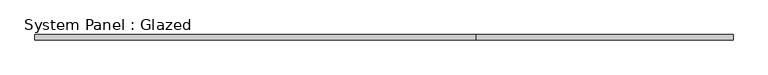
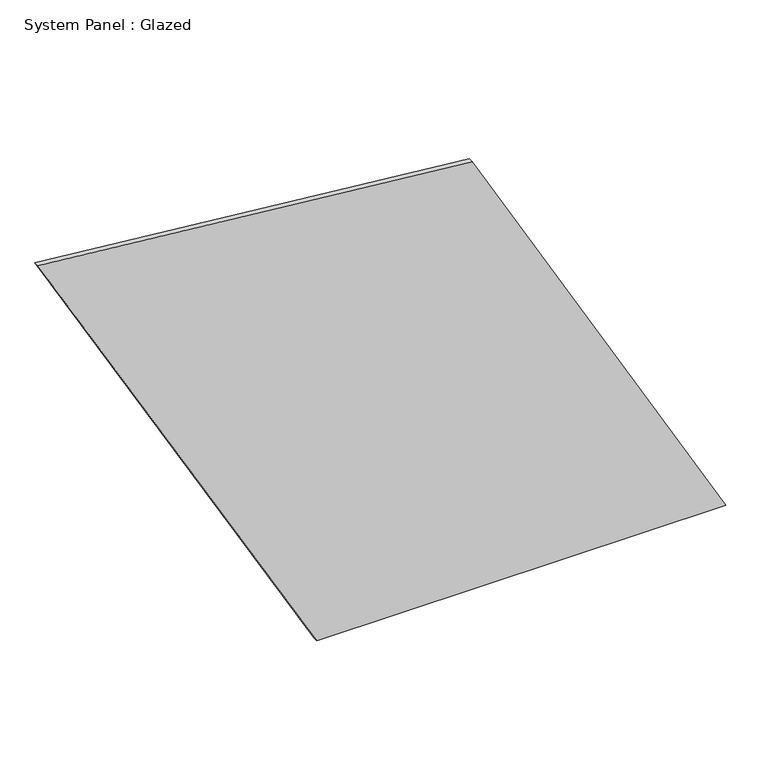
"""IFC4 building model written with IfcOpenShell, lengths in millimetres: plate geometry, System Panel : Glazed."""

from ifc_helpers import new_model, si_unit, frame, origin, place, context, project, spatial, polyline, outline, extrude, source, transform, mapped, element, save


def system_panel_glazed_c7c85ddd(model_context):
    return source(origin(), model_context, "Body", "SweptSolid", [
        extrude(outline(polyline([(0.0, -315.0458616), (0.0, 1662.5416927), (2185.5924268, 436.430046), (2388.6536316, -1662.5416927), (0.0, -315.0458616)])), frame((0.0, -49.5, 0.0), z_axis=(0.0, 1.0, 0.0), x_axis=(0.0, 0.0, 1.0)), (0.0, 0.0, 1.0), 25.0),
    ])


if __name__ == "__main__":
    model = new_model("IFC4")
    model_context = context("Model", 3, world=origin())
    ifc_project = project(units=[si_unit("LENGTHUNIT", "METRE", prefix="MILLI")], contexts=[model_context])
    site = spatial("IfcSite", under=ifc_project)
    building = spatial("IfcBuilding", under=site)
    placement = place(None, origin())
    system_panel_glazed_shape = system_panel_glazed_c7c85ddd(model_context)
    element("IfcPlate", 1, ObjectType="System Panel : Glazed", at=placement, inside=building, context=model_context, shape_type="MappedRepresentation", body=[
        mapped(system_panel_glazed_shape, transform((0.0, 0.0, 0.0), x_axis=(1.0, 0.0, 0.0), y_axis=(0.0, 1.0, 0.0), z_axis=(0.0, 0.0, 1.0))),
    ])
    save(model, "model.ifc")

# Revit data of these elements
# Element 1 (IfcPlate, "System Panel : Glazed")
#   Materials on its faces: "Glass, Clear Glazing"
# Materials
#   "Glass, Clear Glazing": class "Glass", colour RGB 247 249 248, transparency 0.85, Description = "Clear glazing", Cost = 0
